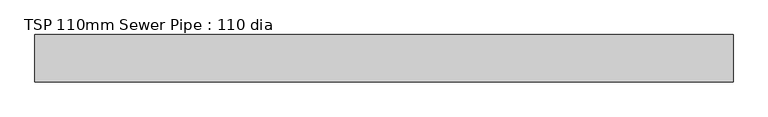
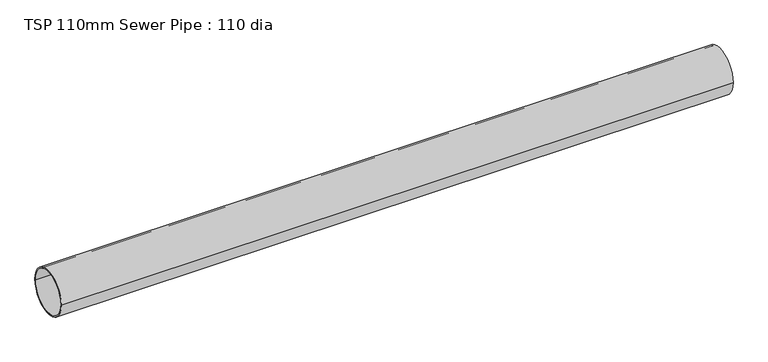
"""IFC4 building model written with IfcOpenShell, lengths in millimetres: flow terminal geometry, TSP 110mm Sewer Pipe : 110 dia."""

from ifc_helpers import new_model, si_unit, point, frame, origin, origin_2d, place, context, project, spatial, circle_curve, trimmed, segment, composite_curve, outline, extrude, source, transform, mapped, element, save


def tsp_110mm_sewer_pipe_110_dia_4c69a6b8(model_context):
    return source(origin(), model_context, "Body", "SweptSolid", [
        extrude(outline(composite_curve([segment(trimmed(circle_curve(origin_2d(), 55.0), [point((-55.0, 0.0))], [point((55.0, 0.0))], False, "CARTESIAN"), True, "CONTINUOUS"), segment(trimmed(circle_curve(origin_2d(), 55.0), [point((55.0, 0.0))], [point((-55.0, 0.0))], False, "CARTESIAN"), True, "CONTINUOUS")], self_intersect=False), holes=[composite_curve([segment(trimmed(circle_curve(origin_2d(), 52.0), [point((-52.0, 0.0))], [point((52.0, 0.0))], True, "CARTESIAN"), True, "CONTINUOUS"), segment(trimmed(circle_curve(origin_2d(), 52.0), [point((52.0, 0.0))], [point((-52.0, 0.0))], True, "CARTESIAN"), True, "CONTINUOUS")], self_intersect=False)]), frame((0.0, 0.0, 0.0), z_axis=(1.0, 0.0, 0.0), x_axis=(0.0, 1.0, 0.0)), (0.0, 0.0, 1.0), 1620.0),
    ])


if __name__ == "__main__":
    model = new_model("IFC4")
    model_context = context("Model", 3, world=origin())
    ifc_project = project(units=[si_unit("LENGTHUNIT", "METRE", prefix="MILLI")], contexts=[model_context])
    site = spatial("IfcSite", under=ifc_project)
    building = spatial("IfcBuilding", under=site)
    placement = place(None, origin())
    tsp_110mm_sewer_pipe_110_dia_shape = tsp_110mm_sewer_pipe_110_dia_4c69a6b8(model_context)
    element("IfcFlowTerminal", 1, ObjectType="TSP 110mm Sewer Pipe : 110 dia", at=placement, inside=building, context=model_context, shape_type="MappedRepresentation", body=[
        mapped(tsp_110mm_sewer_pipe_110_dia_shape, transform((0.0, 0.0, 0.0), x_axis=(1.0, 0.0, 0.0), y_axis=(0.0, 1.0, 0.0), z_axis=(0.0, 0.0, 1.0))),
    ])
    save(model, "model.ifc")

# Revit data of these elements
# Type "TSP 110mm Sewer Pipe : 110 dia"
#   Model = "TSP_110SWB"
#   Model = "TSP_110SWB"
#   Pipe length [instance default] = 1200 mm
#   Pipe dia = 110 mm
#   built-in parameter 1001306 [instance default] = 3.93701 (stored number, unit not read)
#   Default Elevation = 0
# Element 1 (IfcFlowTerminal, "TSP 110mm Sewer Pipe : 110 dia")
#   Pipe length = 1620 mm
#   built-in parameter 1001306 = 5.31496 (stored number, unit not read)
#   Materials on its faces: "Laminate, Brown, Matte"
# Materials
#   "Laminate, Brown, Matte": class "Plastic", colour RGB 128 64 0, transparency 0, Description = "Plastic Laminate - Red, Matte", Cost = 0
